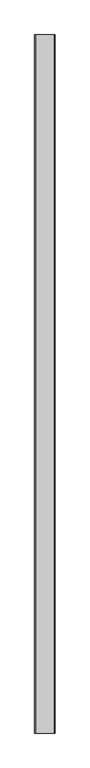
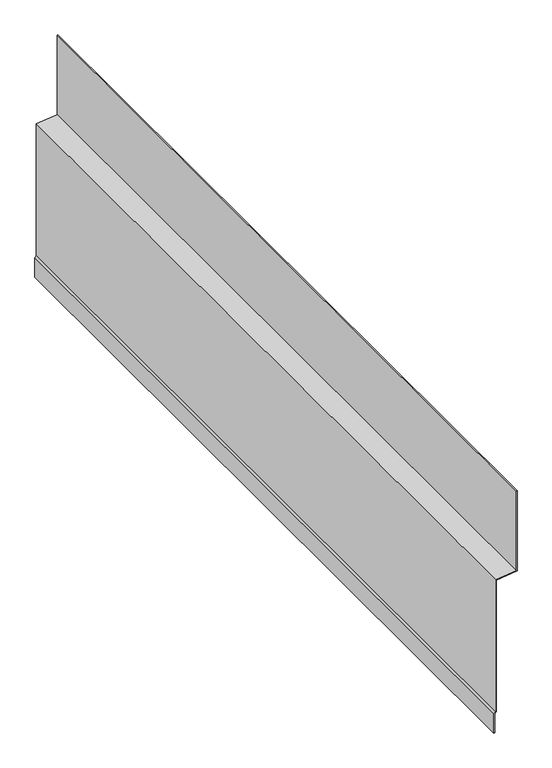
"""IFC4 building model written with IfcOpenShell, lengths in millimetres: proxy geometry, Membrane076 6224 : Membrane076 6224."""

from ifc_helpers import new_model, si_unit, frame, origin, place, context, project, spatial, polyline, outline, extrude, source, transform, mapped, element, save


def generic_models_16bd9644(model_context):
    return source(origin(), model_context, "Body", "SweptSolid", [
        extrude(outline(polyline([(37466.8903328, 10094.1784173), (37255.5079304, 10094.1784173), (37249.3712117, 10041.5599609), (36898.7788361, 10041.5599609), (36895.0835236, 10037.6576172), (36843.396, 10037.6576172), (36843.396, 10039.0576172), (36894.4811548, 10039.0576172), (36898.1764673, 10042.9599609), (37248.125, 10042.9599609), (37254.2617188, 10095.5784173), (37466.8903328, 10095.5784173), (37466.8903328, 10094.1784173)])), frame((0.0, 2217.3609988, 0.0), z_axis=(0.0, 1.0, 0.0), x_axis=(0.0, 0.0, 1.0)), (0.0, 0.0, 1.0), 2000.0),
    ])


if __name__ == "__main__":
    model = new_model("IFC4")
    model_context = context("Model", 3, world=origin())
    ifc_project = project(units=[si_unit("LENGTHUNIT", "METRE", prefix="MILLI")], contexts=[model_context])
    site = spatial("IfcSite", under=ifc_project)
    building = spatial("IfcBuilding", under=site)
    placement = place(None, origin())
    generic_models_shape = generic_models_16bd9644(model_context)
    element("IfcBuildingElementProxy", 1, Name="Membrane076 6224 : Membrane076 6224", ObjectType="Membrane076 6224 : Membrane076 6224", at=placement, inside=building, context=model_context, shape_type="MappedRepresentation", body=[
        mapped(generic_models_shape, transform((0.0, 0.0, 0.0), x_axis=(1.0, 0.0, 0.0), y_axis=(0.0, 1.0, 0.0), z_axis=(0.0, 0.0, 1.0))),
    ])
    save(model, "model.ifc")

# Revit data of these elements
# Type "Membrane076 6224 : Membrane076 6224"
#   NameOverride = "Membrane076"
# Element 1 (IfcBuildingElementProxy, "Membrane076 6224 : Membrane076 6224")
#   Materials on its faces: "(2) LAYERS OF ICE & WATER SHIELD (BITUTHANE) UNDER STUCCO"
# Materials
#   "(2) LAYERS OF ICE & WATER SHIELD (BITUTHANE) UNDER STUCCO": class "Unassigned", colour RGB 186 255 159, transparency 0, Cost = 0
